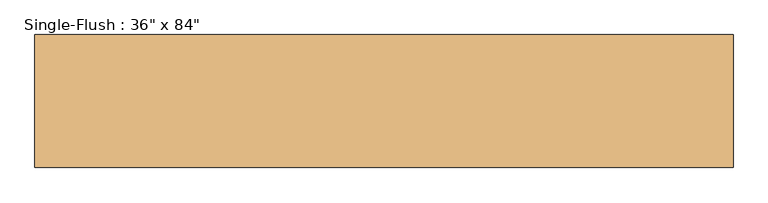
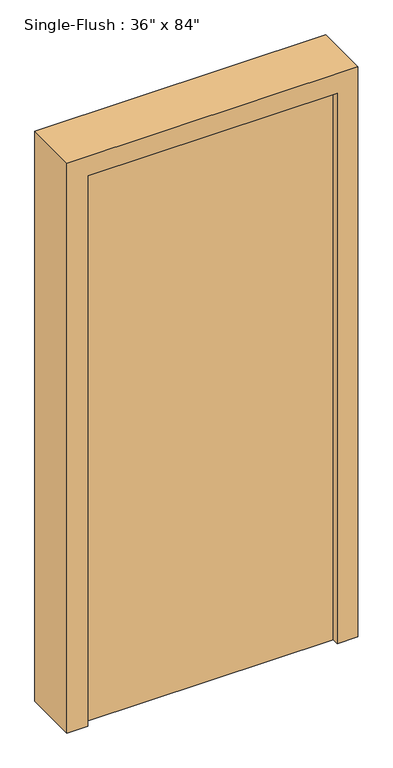
"""IFC4 building model written with IfcOpenShell, lengths in millimetres: door geometry."""

import ifcopenshell
import ifcopenshell.guid

model = None  # the IFC model being written
_history = None  # IfcOwnerHistory: only IFC2X3 demands one
_inside = {}  # id of a spatial element -> (the spatial element, [elements in it])
_under = {}  # id of a project, library or spatial element -> (it, [spatial elements below it])
_declared = {}  # id of a project -> (the project, [libraries it declares])
_typed = {}  # id of a type object -> (the type object, [elements of that type])
_made_of = {}  # id of a material, layer set ... -> (it, [elements and type objects made of it])


def new_model(schema):
    """Start an empty IFC model of exactly this schema.

    Asked for "IFC4X3", IfcOpenShell would pick the latest addendum, in which some entities
    have other attributes; the version numbers below select the first issue.
    IFC2X3 requires an IfcOwnerHistory on every rooted entity: one is made here for all.
    """
    global model, _history
    if schema == "IFC4X3":
        model = ifcopenshell.file(schema_version=(4, 3, 0, 0))
    else:
        model = ifcopenshell.file(schema=schema)
    _inside.clear()
    _under.clear()
    _declared.clear()
    _typed.clear()
    _made_of.clear()
    _history = None
    if model.schema == "IFC2X3":
        org = make("IfcOrganization", Name="unknown")
        user = make(
            "IfcPersonAndOrganization",
            ThePerson=make("IfcPerson", FamilyName="unknown"),
            TheOrganization=org,
        )
        app = make(
            "IfcApplication",
            ApplicationDeveloper=org,
            Version="unknown",
            ApplicationFullName="unknown",
            ApplicationIdentifier="unknown",
        )
        _history = make(
            "IfcOwnerHistory",
            OwningUser=user,
            OwningApplication=app,
            ChangeAction="ADDED",
            CreationDate=0,
        )
    return model


def make(cls, **values):
    """One entity of the class cls with the attributes given. An attribute that is None is left unset."""
    return model.create_entity(
        cls, **{name: value for name, value in values.items() if value is not None}
    )


def rooted(cls, **values):
    """An entity with a GlobalId (a new one), such as an element, a storey or a relation."""
    return make(cls, GlobalId=ifcopenshell.guid.new(), OwnerHistory=_history, **values)


def si_unit(unit_type, name, prefix=None):
    """IfcSIUnit, for example si_unit("LENGTHUNIT", "METRE", prefix="MILLI")."""
    return make("IfcSIUnit", UnitType=unit_type, Prefix=prefix, Name=name)


def assignment(units):
    """IfcUnitAssignment: the units of a project."""
    return None if units is None else make("IfcUnitAssignment", Units=units)


def point(xyz):
    """IfcCartesianPoint."""
    return None if xyz is None else make("IfcCartesianPoint", Coordinates=xyz)


def direction(xyz):
    """IfcDirection."""
    return None if xyz is None else make("IfcDirection", DirectionRatios=xyz)


def frame(location, z_axis=None, x_axis=None):
    """IfcAxis2Placement3D, a coordinate frame: its origin and axes. An axis left out is left unset."""
    return make(
        "IfcAxis2Placement3D",
        Location=point(location),
        Axis=direction(z_axis),
        RefDirection=direction(x_axis),
    )


def origin():
    """The frame at (0, 0, 0) with its axes left unset."""
    return frame((0.0, 0.0, 0.0))


def origin_with_axes():
    """The frame at (0, 0, 0) with the z axis (0, 0, 1) and the x axis (1, 0, 0) written out."""
    return frame((0.0, 0.0, 0.0), z_axis=(0.0, 0.0, 1.0), x_axis=(1.0, 0.0, 0.0))


def place(relative_to, where):
    """IfcLocalPlacement: puts the frame where relative to a parent placement (None: the world)."""
    return make(
        "IfcLocalPlacement", PlacementRelTo=relative_to, RelativePlacement=where
    )


def context(
    kind, dimensions, precision=None, world=None, true_north=None, identifier=None
):
    """IfcGeometricRepresentationContext, for example the 3D "Model" context."""
    return make(
        "IfcGeometricRepresentationContext",
        ContextIdentifier=identifier,
        ContextType=kind,
        CoordinateSpaceDimension=dimensions,
        Precision=precision,
        WorldCoordinateSystem=world,
        TrueNorth=true_north,
    )


def project(units=None, contexts=None):
    """IfcProject with its units and contexts."""
    return rooted(
        "IfcProject",
        Name="project",
        RepresentationContexts=contexts,
        UnitsInContext=assignment(units),
    )


def spatial(cls, under=None, at=None, **own):
    """A site, building, storey or space (cls), placed at a placement, below another one or the project."""
    s = rooted(cls, ObjectPlacement=at, **own)
    if under is not None:
        _under.setdefault(under.id(), (under, []))[1].append(s)
    return s


def polyline(points):
    """IfcPolyline through the points."""
    return make("IfcPolyline", Points=[point(p) for p in points])


def outline(outer, holes=None, kind="AREA"):
    """IfcArbitraryClosedProfileDef: a profile drawn as a closed curve; with holes, ...WithVoids."""
    if holes is None:
        return make("IfcArbitraryClosedProfileDef", ProfileType=kind, OuterCurve=outer)
    return make(
        "IfcArbitraryProfileDefWithVoids",
        ProfileType=kind,
        OuterCurve=outer,
        InnerCurves=holes,
    )


def extrude(swept, where, along, depth):
    """IfcExtrudedAreaSolid: the profile swept, set in the frame where, extruded along a direction by depth."""
    return make(
        "IfcExtrudedAreaSolid",
        SweptArea=swept,
        Position=where,
        ExtrudedDirection=direction(along),
        Depth=depth,
    )


def shape(context_of_items, identifier, shape_type, items):
    """IfcShapeRepresentation: the items that make up one representation, for example the "Body"."""
    return make(
        "IfcShapeRepresentation",
        ContextOfItems=context_of_items,
        RepresentationIdentifier=identifier,
        RepresentationType=shape_type,
        Items=items,
    )


def source(mapping_origin, context_of_items, identifier, shape_type, items):
    """IfcRepresentationMap: a shape defined once, which mapped items show again and again."""
    return make(
        "IfcRepresentationMap",
        MappingOrigin=mapping_origin,
        MappedRepresentation=shape(context_of_items, identifier, shape_type, items),
    )


def transform(
    local_origin,
    x_axis=None,
    y_axis=None,
    z_axis=None,
    scale=None,
    scale2=None,
    scale3=None,
    uniform=True,
):
    """IfcCartesianTransformationOperator3D, or its non-uniform kind. x_axis, y_axis, z_axis: its Axis1, 2, 3."""
    if uniform:
        return make(
            "IfcCartesianTransformationOperator3D",
            Axis1=direction(x_axis),
            Axis2=direction(y_axis),
            LocalOrigin=point(local_origin),
            Scale=scale,
            Axis3=direction(z_axis),
        )
    return make(
        "IfcCartesianTransformationOperator3DnonUniform",
        Axis1=direction(x_axis),
        Axis2=direction(y_axis),
        LocalOrigin=point(local_origin),
        Scale=scale,
        Axis3=direction(z_axis),
        Scale2=scale2,
        Scale3=scale3,
    )


def mapped(mapping_source, mapping_target):
    """IfcMappedItem: shows the shape of a source again, moved by a transform."""
    return make(
        "IfcMappedItem", MappingSource=mapping_source, MappingTarget=mapping_target
    )


def made_of(thing, what):
    """Note that an element or type object is made of a material, layer set ...; save() writes the relation."""
    if what is not None:
        _made_of.setdefault(what.id(), (what, []))[1].append(thing)
    return thing


def element(
    cls,
    number,
    at=None,
    inside=None,
    cuts=None,
    type_object=None,
    material=None,
    context=None,
    identifier="Body",
    shape_type=None,
    held_by="IfcProductDefinitionShape",
    body=None,
    shapes=None,
    **own,
):
    """One element of the class cls, such as IfcWall. Its Tag is "e" and its number.

    at: its placement. inside: the storey or other place that contains it. cuts: it is an
    opening in that element (IfcRelVoidsElement). A single representation is given by context,
    identifier, shape_type and body (its items); several are given by shapes. held_by: the class
    of the entity that holds the representations. save() writes the other relations.
    """
    e = rooted(cls, Tag="e%d" % number, ObjectPlacement=at, **own)
    if body is not None:
        shapes = [shape(context, identifier, shape_type, body)]
    if shapes is not None:
        e.Representation = make(held_by, Representations=shapes)
    if inside is not None:
        _inside.setdefault(inside.id(), (inside, []))[1].append(e)
    if cuts is not None:
        rooted(
            "IfcRelVoidsElement", RelatingBuildingElement=cuts, RelatedOpeningElement=e
        )
    if type_object is not None:
        _typed.setdefault(type_object.id(), (type_object, []))[1].append(e)
    return made_of(e, material)


def aggregate(whole, parts):
    """IfcRelAggregates: a whole, such as a stair, and the parts it consists of."""
    return rooted("IfcRelAggregates", RelatingObject=whole, RelatedObjects=parts)


def save(model, path):
    """Write the relations noted so far, then the file.

    IfcRelAggregates (storeys below a building ...), IfcRelContainedInSpatialStructure (elements
    in a storey), IfcRelDefinesByType, IfcRelAssociatesMaterial and IfcRelDeclares: one each for
    every whole, place, type object, material and project.
    """
    for whole, parts in _under.values():
        aggregate(whole, parts)
    for where, things in _inside.values():
        rooted(
            "IfcRelContainedInSpatialStructure",
            RelatedElements=things,
            RelatingStructure=where,
        )
    for kind, things in _typed.values():
        rooted("IfcRelDefinesByType", RelatedObjects=things, RelatingType=kind)
    for what, things in _made_of.values():
        rooted("IfcRelAssociatesMaterial", RelatedObjects=things, RelatingMaterial=what)
    for by, libraries in _declared.values():
        rooted("IfcRelDeclares", RelatingContext=by, RelatedDefinitions=libraries)
    model.write(path)


def door_983db92c(model_context):
    return source(origin(), model_context, "Body", "SweptSolid", [
        extrude(outline(polyline([(2209.8, 533.4), (2209.8, -533.4), (0.0, -533.4), (0.0, -457.2), (2133.6, -457.2), (2133.6, 457.2), (0.0, 457.2), (0.0, 533.4), (2209.8, 533.4)])), frame((0.0, -101.6, 0.0), z_axis=(0.0, 1.0, 0.0), x_axis=(0.0, 0.0, 1.0)), (0.0, 0.0, 1.0), 203.2),
        extrude(outline(polyline([(457.2, -25.4), (457.2, -76.2), (-457.2, -76.2), (-457.2, -25.4), (457.2, -25.4)])), origin_with_axes(), (0.0, 0.0, 1.0), 2133.6),
    ])


if __name__ == "__main__":
    model = new_model("IFC4")
    model_context = context("Model", 3, world=origin())
    ifc_project = project(units=[si_unit("LENGTHUNIT", "METRE", prefix="MILLI")], contexts=[model_context])
    site = spatial("IfcSite", under=ifc_project)
    building = spatial("IfcBuilding", under=site)
    placement = place(None, origin())
    door_shape = door_983db92c(model_context)
    element("IfcDoor", 1, ObjectType="Single-Flush : 36\" x 84\"", at=placement, inside=building, context=model_context, shape_type="MappedRepresentation", body=[
        mapped(door_shape, transform((0.0, 0.0, 0.0), x_axis=(1.0, 0.0, 0.0), y_axis=(0.0, 1.0, 0.0), z_axis=(0.0, 0.0, 1.0))),
    ])
    save(model, "model.ifc")

# Revit data of these elements
# Type "Single-Flush : 36\" x 84\""
#   Type Mark = "40"
#   Construction Type Id = "MDOOR"
#   Assembly Code = "C1020"
#   Analytic Construction = "Metal"
#   Thickness = 0' - 2"
#   Thermal Resistance (R) = 0.270117 (m²·K)/W
#   Heat Transfer Coefficient (U) = 3.7021 W/(m²·K)
#   Height = 7' - 0"
#   Trim Projection Ext = 0' - 1"
#   Trim Projection Int = 0' - 1"
#   Trim Width = 0' - 3"
#   Width = 3' - 0"
#   Door Material = Door - Panel
#   Frame Material = Door - Frame
#   Visual Light Transmittance = 0
#   Solar Heat Gain Coefficient = 0
#   Function = (empty or 0)
#   Wall Closure = (empty or 0)
# Element 1 (IfcDoor, "Single-Flush : 36\" x 84\"")
#   Materials on its faces: "Door - Frame", "Door - Panel"
# Materials
#   "Door - Panel": class "Wood", colour RGB 212 179 113, transparency 0, Cost = 0
#   "Door - Frame": class "Miscellaneous", colour RGB 65 65 65, transparency 0, Cost = 0
